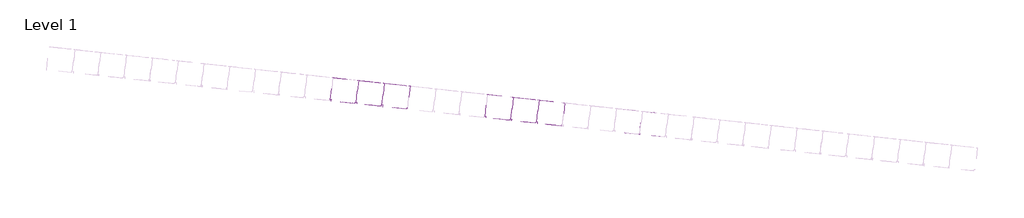
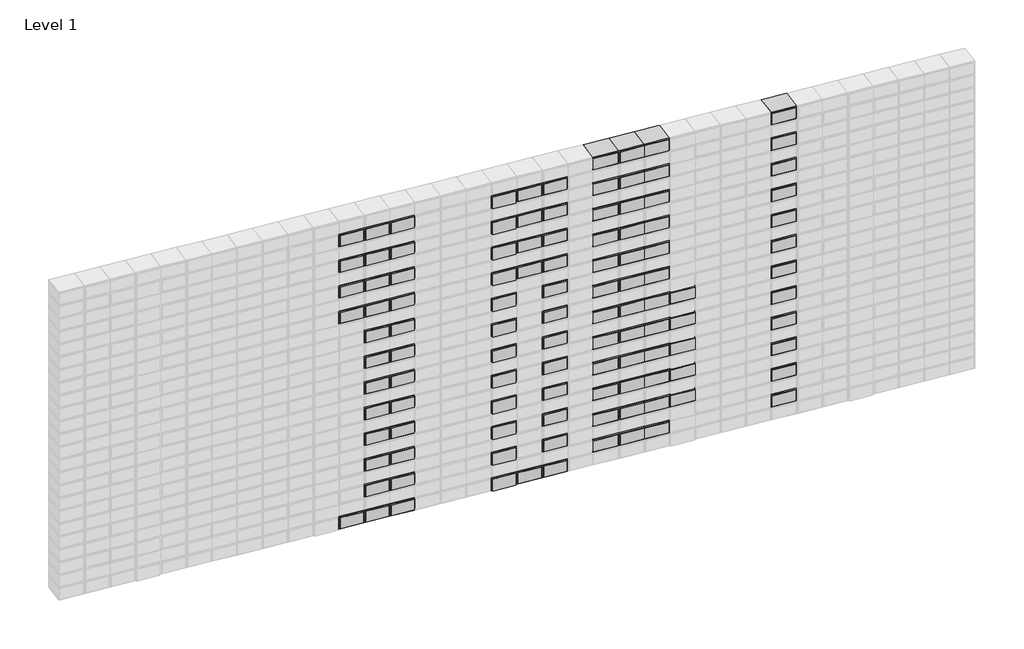
# One storey, part 15 of 18: 111 proxies.
"""IFC4 building model written with IfcOpenShell, lengths in millimetres."""

import ifcopenshell
import ifcopenshell.guid

model = None  # the IFC model being written
_history = None  # IfcOwnerHistory: only IFC2X3 demands one
_inside = {}  # id of a spatial element -> (the spatial element, [elements in it])
_under = {}  # id of a project, library or spatial element -> (it, [spatial elements below it])
_declared = {}  # id of a project -> (the project, [libraries it declares])
_typed = {}  # id of a type object -> (the type object, [elements of that type])
_made_of = {}  # id of a material, layer set ... -> (it, [elements and type objects made of it])


def new_model(schema):
    """Start an empty IFC model of exactly this schema.

    Asked for "IFC4X3", IfcOpenShell would pick the latest addendum, in which some entities
    have other attributes; the version numbers below select the first issue.
    IFC2X3 requires an IfcOwnerHistory on every rooted entity: one is made here for all.
    """
    global model, _history
    if schema == "IFC4X3":
        model = ifcopenshell.file(schema_version=(4, 3, 0, 0))
    else:
        model = ifcopenshell.file(schema=schema)
    _inside.clear()
    _under.clear()
    _declared.clear()
    _typed.clear()
    _made_of.clear()
    _history = None
    if model.schema == "IFC2X3":
        org = make("IfcOrganization", Name="unknown")
        user = make(
            "IfcPersonAndOrganization",
            ThePerson=make("IfcPerson", FamilyName="unknown"),
            TheOrganization=org,
        )
        app = make(
            "IfcApplication",
            ApplicationDeveloper=org,
            Version="unknown",
            ApplicationFullName="unknown",
            ApplicationIdentifier="unknown",
        )
        _history = make(
            "IfcOwnerHistory",
            OwningUser=user,
            OwningApplication=app,
            ChangeAction="ADDED",
            CreationDate=0,
        )
    return model


def make(cls, **values):
    """One entity of the class cls with the attributes given. An attribute that is None is left unset."""
    return model.create_entity(
        cls, **{name: value for name, value in values.items() if value is not None}
    )


def rooted(cls, **values):
    """An entity with a GlobalId (a new one), such as an element, a storey or a relation."""
    return make(cls, GlobalId=ifcopenshell.guid.new(), OwnerHistory=_history, **values)


def si_unit(unit_type, name, prefix=None):
    """IfcSIUnit, for example si_unit("LENGTHUNIT", "METRE", prefix="MILLI")."""
    return make("IfcSIUnit", UnitType=unit_type, Prefix=prefix, Name=name)


def assignment(units):
    """IfcUnitAssignment: the units of a project."""
    return None if units is None else make("IfcUnitAssignment", Units=units)


def point(xyz):
    """IfcCartesianPoint."""
    return None if xyz is None else make("IfcCartesianPoint", Coordinates=xyz)


def direction(xyz):
    """IfcDirection."""
    return None if xyz is None else make("IfcDirection", DirectionRatios=xyz)


def frame(location, z_axis=None, x_axis=None):
    """IfcAxis2Placement3D, a coordinate frame: its origin and axes. An axis left out is left unset."""
    return make(
        "IfcAxis2Placement3D",
        Location=point(location),
        Axis=direction(z_axis),
        RefDirection=direction(x_axis),
    )


def origin():
    """The frame at (0, 0, 0) with its axes left unset."""
    return frame((0.0, 0.0, 0.0))


def origin_with_axes():
    """The frame at (0, 0, 0) with the z axis (0, 0, 1) and the x axis (1, 0, 0) written out."""
    return frame((0.0, 0.0, 0.0), z_axis=(0.0, 0.0, 1.0), x_axis=(1.0, 0.0, 0.0))


def place(relative_to, where):
    """IfcLocalPlacement: puts the frame where relative to a parent placement (None: the world)."""
    return make(
        "IfcLocalPlacement", PlacementRelTo=relative_to, RelativePlacement=where
    )


def context(
    kind, dimensions, precision=None, world=None, true_north=None, identifier=None
):
    """IfcGeometricRepresentationContext, for example the 3D "Model" context."""
    return make(
        "IfcGeometricRepresentationContext",
        ContextIdentifier=identifier,
        ContextType=kind,
        CoordinateSpaceDimension=dimensions,
        Precision=precision,
        WorldCoordinateSystem=world,
        TrueNorth=true_north,
    )


def project(units=None, contexts=None):
    """IfcProject with its units and contexts."""
    return rooted(
        "IfcProject",
        Name="project",
        RepresentationContexts=contexts,
        UnitsInContext=assignment(units),
    )


def spatial(cls, under=None, at=None, **own):
    """A site, building, storey or space (cls), placed at a placement, below another one or the project."""
    s = rooted(cls, ObjectPlacement=at, **own)
    if under is not None:
        _under.setdefault(under.id(), (under, []))[1].append(s)
    return s


def polyline(points):
    """IfcPolyline through the points."""
    return make("IfcPolyline", Points=[point(p) for p in points])


def outline(outer, holes=None, kind="AREA"):
    """IfcArbitraryClosedProfileDef: a profile drawn as a closed curve; with holes, ...WithVoids."""
    if holes is None:
        return make("IfcArbitraryClosedProfileDef", ProfileType=kind, OuterCurve=outer)
    return make(
        "IfcArbitraryProfileDefWithVoids",
        ProfileType=kind,
        OuterCurve=outer,
        InnerCurves=holes,
    )


def extrude(swept, where, along, depth):
    """IfcExtrudedAreaSolid: the profile swept, set in the frame where, extruded along a direction by depth."""
    return make(
        "IfcExtrudedAreaSolid",
        SweptArea=swept,
        Position=where,
        ExtrudedDirection=direction(along),
        Depth=depth,
    )


def shape(context_of_items, identifier, shape_type, items):
    """IfcShapeRepresentation: the items that make up one representation, for example the "Body"."""
    return make(
        "IfcShapeRepresentation",
        ContextOfItems=context_of_items,
        RepresentationIdentifier=identifier,
        RepresentationType=shape_type,
        Items=items,
    )


def source(mapping_origin, context_of_items, identifier, shape_type, items):
    """IfcRepresentationMap: a shape defined once, which mapped items show again and again."""
    return make(
        "IfcRepresentationMap",
        MappingOrigin=mapping_origin,
        MappedRepresentation=shape(context_of_items, identifier, shape_type, items),
    )


def transform(
    local_origin,
    x_axis=None,
    y_axis=None,
    z_axis=None,
    scale=None,
    scale2=None,
    scale3=None,
    uniform=True,
):
    """IfcCartesianTransformationOperator3D, or its non-uniform kind. x_axis, y_axis, z_axis: its Axis1, 2, 3."""
    if uniform:
        return make(
            "IfcCartesianTransformationOperator3D",
            Axis1=direction(x_axis),
            Axis2=direction(y_axis),
            LocalOrigin=point(local_origin),
            Scale=scale,
            Axis3=direction(z_axis),
        )
    return make(
        "IfcCartesianTransformationOperator3DnonUniform",
        Axis1=direction(x_axis),
        Axis2=direction(y_axis),
        LocalOrigin=point(local_origin),
        Scale=scale,
        Axis3=direction(z_axis),
        Scale2=scale2,
        Scale3=scale3,
    )


def mapped(mapping_source, mapping_target):
    """IfcMappedItem: shows the shape of a source again, moved by a transform."""
    return make(
        "IfcMappedItem", MappingSource=mapping_source, MappingTarget=mapping_target
    )


def made_of(thing, what):
    """Note that an element or type object is made of a material, layer set ...; save() writes the relation."""
    if what is not None:
        _made_of.setdefault(what.id(), (what, []))[1].append(thing)
    return thing


def element(
    cls,
    number,
    at=None,
    inside=None,
    cuts=None,
    type_object=None,
    material=None,
    context=None,
    identifier="Body",
    shape_type=None,
    held_by="IfcProductDefinitionShape",
    body=None,
    shapes=None,
    **own,
):
    """One element of the class cls, such as IfcWall. Its Tag is "e" and its number.

    at: its placement. inside: the storey or other place that contains it. cuts: it is an
    opening in that element (IfcRelVoidsElement). A single representation is given by context,
    identifier, shape_type and body (its items); several are given by shapes. held_by: the class
    of the entity that holds the representations. save() writes the other relations.
    """
    e = rooted(cls, Tag="e%d" % number, ObjectPlacement=at, **own)
    if body is not None:
        shapes = [shape(context, identifier, shape_type, body)]
    if shapes is not None:
        e.Representation = make(held_by, Representations=shapes)
    if inside is not None:
        _inside.setdefault(inside.id(), (inside, []))[1].append(e)
    if cuts is not None:
        rooted(
            "IfcRelVoidsElement", RelatingBuildingElement=cuts, RelatedOpeningElement=e
        )
    if type_object is not None:
        _typed.setdefault(type_object.id(), (type_object, []))[1].append(e)
    return made_of(e, material)


def aggregate(whole, parts):
    """IfcRelAggregates: a whole, such as a stair, and the parts it consists of."""
    return rooted("IfcRelAggregates", RelatingObject=whole, RelatedObjects=parts)


def save(model, path):
    """Write the relations noted so far, then the file.

    IfcRelAggregates (storeys below a building ...), IfcRelContainedInSpatialStructure (elements
    in a storey), IfcRelDefinesByType, IfcRelAssociatesMaterial and IfcRelDeclares: one each for
    every whole, place, type object, material and project.
    """
    for whole, parts in _under.values():
        aggregate(whole, parts)
    for where, things in _inside.values():
        rooted(
            "IfcRelContainedInSpatialStructure",
            RelatedElements=things,
            RelatingStructure=where,
        )
    for kind, things in _typed.values():
        rooted("IfcRelDefinesByType", RelatedObjects=things, RelatingType=kind)
    for what, things in _made_of.values():
        rooted("IfcRelAssociatesMaterial", RelatedObjects=things, RelatingMaterial=what)
    for by, libraries in _declared.values():
        rooted("IfcRelDeclares", RelatingContext=by, RelatedDefinitions=libraries)
    model.write(path)


def geel_a5fc7152(model_context):
    return source(origin(), model_context, "Body", "SweptSolid", [
        extrude(outline(polyline([(131.1871262, 51.8695461), (24.8461542, 24.0369432), (23.5801491, 28.8740117), (125.0840527, 55.4406095), (111.9430518, 105.6488784), (10.4391482, 79.0822806), (9.1731432, 83.919349), (115.5141152, 111.7519519), (131.1871262, 51.8695461)])), origin_with_axes(), (0.0, 0.0, 1.0), 95.0),
        extrude(outline(polyline([(111.9430518, 105.6488784), (125.0840527, 55.4406095), (23.5801491, 28.8740117), (10.4391482, 79.0822806), (111.9430518, 105.6488784)])), origin_with_axes(), (0.0, 0.0, 1.0), 100.0),
    ])


def geel_ff5a4212(model_context):
    return source(origin(), model_context, "Body", "SweptSolid", [
        extrude(outline(polyline([(24.8461542, 24.0369432), (9.1731432, 83.919349), (115.5141152, 111.7519519), (116.7801202, 106.9148835), (15.2762167, 80.3482856), (28.4172176, 30.1400167), (129.9211211, 56.7066146), (131.1871262, 51.8695461), (24.8461542, 24.0369432)])), origin_with_axes(), (0.0, 0.0, 1.0), 95.0),
        extrude(outline(polyline([(116.7801202, 106.9148835), (129.9211211, 56.7066146), (28.4172176, 30.1400167), (15.2762167, 80.3482856), (116.7801202, 106.9148835)])), origin_with_axes(), (0.0, 0.0, 1.0), 100.0),
    ])


def rood_14a66368(model_context):
    return source(origin(), model_context, "Body", "SweptSolid", [
        extrude(outline(polyline([(24.8461542, 24.0369432), (9.1731432, 83.919349), (115.5141152, 111.7519519), (131.1871262, 51.8695461), (24.8461542, 24.0369432)]), holes=[polyline([(125.0840527, 55.4406095), (111.9430518, 105.6488784), (15.2762167, 80.3482856), (28.4172176, 30.1400167), (125.0840527, 55.4406095)])]), origin_with_axes(), (0.0, 0.0, 1.0), 95.0),
        extrude(outline(polyline([(111.9430518, 105.6488784), (125.0840527, 55.4406095), (28.4172176, 30.1400167), (15.2762167, 80.3482856), (111.9430518, 105.6488784)])), origin_with_axes(), (0.0, 0.0, 1.0), 100.0),
    ])


def rood_2ddd8018(model_context):
    return source(origin(), model_context, "Body", "SweptSolid", [
        extrude(outline(polyline([(24.8461542, 24.0369432), (9.1731432, 83.919349), (115.5141152, 111.7519519), (131.1871262, 51.8695461), (126.3500577, 50.6035411), (111.9430518, 105.6488784), (15.2762167, 80.3482856), (29.6832226, 25.3029482), (24.8461542, 24.0369432)])), origin_with_axes(), (0.0, 0.0, 1.0), 95.0),
        extrude(outline(polyline([(111.9430518, 105.6488784), (126.3500577, 50.6035411), (29.6832226, 25.3029482), (15.2762167, 80.3482856), (111.9430518, 105.6488784)])), origin_with_axes(), (0.0, 0.0, 1.0), 100.0),
    ])


model = new_model("IFC4")

# Units and contexts
model_context = context("Model", 3, world=origin())
ifc_project = project(units=[si_unit("LENGTHUNIT", "METRE", prefix="MILLI")], contexts=[model_context])

# Site, building, storey
site = spatial("IfcSite", under=ifc_project)
building = spatial("IfcBuilding", under=site)
storey = spatial("IfcBuildingStorey", under=building, Name="Level 1", Elevation=0.0)

# Proxies
placement = place(None, origin())
geel_shape = geel_a5fc7152(model_context)
element("IfcBuildingElementProxy", 1, Name="Geel", ObjectType="Geel", at=placement, inside=storey, context=model_context, shape_type="MappedRepresentation", body=[
    mapped(geel_shape, transform((11171.9037428, -4526.1762984, 2168.7358475), x_axis=(0.9617275503729374, -0.1047347566147725, -0.25320100633787673), y_axis=(0.25171277368869216, -0.02741220845642974, 0.9674136914420255), z_axis=(-0.10826263628609081, -0.9941223272738551, 0.0))),
])
element("IfcBuildingElementProxy", 2, Name="Geel", ObjectType="Geel", at=placement, inside=storey, context=model_context, shape_type="MappedRepresentation", body=[
    mapped(geel_shape, transform((11936.8417921, -4609.4801409, 2168.7358475), x_axis=(0.9617275503729374, -0.10473475661477244, -0.25320100633787673), y_axis=(0.25171277368869216, -0.027412208456429728, 0.9674136914420255), z_axis=(-0.10826263628609079, -0.9941223272738551, 0.0))),
])
element("IfcBuildingElementProxy", 3, Name="Geel", ObjectType="Geel", at=placement, inside=storey, context=model_context, shape_type="MappedRepresentation", body=[
    mapped(geel_shape, transform((11171.9037428, -4526.1762984, 2292.5348104), x_axis=(0.9617275503729374, -0.1047347566147725, -0.25320100633787673), y_axis=(0.25171277368869216, -0.02741220845642974, 0.9674136914420255), z_axis=(-0.10826263628609081, -0.9941223272738551, 0.0))),
])
element("IfcBuildingElementProxy", 4, Name="Geel", ObjectType="Geel", at=placement, inside=storey, context=model_context, shape_type="MappedRepresentation", body=[
    mapped(geel_shape, transform((11936.8417921, -4609.4801409, 2292.5348104), x_axis=(0.9617275503729374, -0.10473475661477244, -0.25320100633787673), y_axis=(0.25171277368869216, -0.027412208456429728, 0.9674136914420255), z_axis=(-0.10826263628609079, -0.9941223272738551, 0.0))),
])
element("IfcBuildingElementProxy", 5, Name="Geel", ObjectType="Geel", at=placement, inside=storey, context=model_context, shape_type="MappedRepresentation", body=[
    mapped(geel_shape, transform((11171.9037428, -4526.1762984, 2416.3337732), x_axis=(0.9617275503729384, -0.1047347566147726, -0.25320100633787307), y_axis=(0.25171277368868855, -0.02741220845642934, 0.9674136914420265), z_axis=(-0.10826263628609081, -0.994122327273855, 0.0))),
])
element("IfcBuildingElementProxy", 6, Name="Geel", ObjectType="Geel", at=placement, inside=storey, context=model_context, shape_type="MappedRepresentation", body=[
    mapped(geel_shape, transform((11936.8417921, -4609.4801409, 2416.3337732), x_axis=(0.9617275503729384, -0.10473475661477255, -0.25320100633787307), y_axis=(0.25171277368868855, -0.027412208456429325, 0.9674136914420265), z_axis=(-0.10826263628609077, -0.994122327273855, 0.0))),
])
element("IfcBuildingElementProxy", 7, Name="Geel", ObjectType="Geel", at=placement, inside=storey, context=model_context, shape_type="MappedRepresentation", body=[
    mapped(geel_shape, transform((11171.9037428, -4526.1762984, 2540.132736), x_axis=(0.9617275503729374, -0.1047347566147725, -0.25320100633787673), y_axis=(0.25171277368869216, -0.02741220845642974, 0.9674136914420255), z_axis=(-0.10826263628609081, -0.9941223272738551, 0.0))),
])
element("IfcBuildingElementProxy", 8, Name="Geel", ObjectType="Geel", at=placement, inside=storey, context=model_context, shape_type="MappedRepresentation", body=[
    mapped(geel_shape, transform((11936.8417921, -4609.4801409, 2540.132736), x_axis=(0.9617275503729374, -0.10473475661477244, -0.25320100633787673), y_axis=(0.25171277368869216, -0.027412208456429728, 0.9674136914420255), z_axis=(-0.10826263628609079, -0.9941223272738551, 0.0))),
])
element("IfcBuildingElementProxy", 9, Name="Geel", ObjectType="Geel", at=placement, inside=storey, context=model_context, shape_type="MappedRepresentation", body=[
    mapped(geel_shape, transform((11171.9037428, -4526.1762984, 2663.9316989), x_axis=(0.9617275503729374, -0.1047347566147725, -0.25320100633787673), y_axis=(0.25171277368869216, -0.02741220845642974, 0.9674136914420255), z_axis=(-0.10826263628609081, -0.9941223272738551, 0.0))),
])
element("IfcBuildingElementProxy", 10, Name="Geel", ObjectType="Geel", at=placement, inside=storey, context=model_context, shape_type="MappedRepresentation", body=[
    mapped(geel_shape, transform((11936.8417921, -4609.4801409, 2663.9316989), x_axis=(0.9617275503729374, -0.10473475661477244, -0.25320100633787673), y_axis=(0.25171277368869216, -0.027412208456429728, 0.9674136914420255), z_axis=(-0.10826263628609079, -0.9941223272738551, 0.0))),
])
element("IfcBuildingElementProxy", 11, Name="Geel", ObjectType="Geel", at=placement, inside=storey, context=model_context, shape_type="MappedRepresentation", body=[
    mapped(geel_shape, transform((11171.9037428, -4526.1762984, 2787.7306617), x_axis=(0.9617275503729374, -0.1047347566147725, -0.25320100633787673), y_axis=(0.25171277368869216, -0.02741220845642974, 0.9674136914420255), z_axis=(-0.10826263628609081, -0.9941223272738551, 0.0))),
])
element("IfcBuildingElementProxy", 12, Name="Geel", ObjectType="Geel", at=placement, inside=storey, context=model_context, shape_type="MappedRepresentation", body=[
    mapped(geel_shape, transform((11936.8417921, -4609.4801409, 2787.7306617), x_axis=(0.9617275503729374, -0.10473475661477244, -0.25320100633787673), y_axis=(0.25171277368869216, -0.027412208456429728, 0.9674136914420255), z_axis=(-0.10826263628609079, -0.9941223272738551, 0.0))),
])
element("IfcBuildingElementProxy", 13, Name="Geel", ObjectType="Geel", at=placement, inside=storey, context=model_context, shape_type="MappedRepresentation", body=[
    mapped(geel_shape, transform((11171.9037428, -4526.1762984, 2911.5296245), x_axis=(0.9617275503729374, -0.1047347566147725, -0.25320100633787673), y_axis=(0.25171277368869216, -0.02741220845642974, 0.9674136914420255), z_axis=(-0.10826263628609081, -0.9941223272738551, 0.0))),
])
element("IfcBuildingElementProxy", 14, Name="Geel", ObjectType="Geel", at=placement, inside=storey, context=model_context, shape_type="MappedRepresentation", body=[
    mapped(geel_shape, transform((11936.8417921, -4609.4801409, 2911.5296245), x_axis=(0.9617275503729374, -0.10473475661477244, -0.25320100633787673), y_axis=(0.25171277368869216, -0.027412208456429728, 0.9674136914420255), z_axis=(-0.10826263628609079, -0.9941223272738551, 0.0))),
])
element("IfcBuildingElementProxy", 15, Name="Geel", ObjectType="Geel", at=placement, inside=storey, context=model_context, shape_type="MappedRepresentation", body=[
    mapped(geel_shape, transform((11171.9037428, -4526.1762984, 3035.3285874), x_axis=(0.9617275503729374, -0.1047347566147725, -0.25320100633787673), y_axis=(0.25171277368869216, -0.02741220845642974, 0.9674136914420255), z_axis=(-0.10826263628609081, -0.9941223272738551, 0.0))),
])
element("IfcBuildingElementProxy", 16, Name="Geel", ObjectType="Geel", at=placement, inside=storey, context=model_context, shape_type="MappedRepresentation", body=[
    mapped(geel_shape, transform((11936.8417921, -4609.4801409, 3035.3285874), x_axis=(0.9617275503729374, -0.10473475661477244, -0.25320100633787673), y_axis=(0.25171277368869216, -0.027412208456429728, 0.9674136914420255), z_axis=(-0.10826263628609079, -0.9941223272738551, 0.0))),
])
element("IfcBuildingElementProxy", 17, Name="Geel", ObjectType="Geel", at=placement, inside=storey, context=model_context, shape_type="MappedRepresentation", body=[
    mapped(geel_shape, transform((11171.9037428, -4526.1762984, 3159.1275502), x_axis=(0.9617275503729374, -0.1047347566147725, -0.25320100633787673), y_axis=(0.25171277368869216, -0.02741220845642974, 0.9674136914420255), z_axis=(-0.10826263628609081, -0.9941223272738551, 0.0))),
])
element("IfcBuildingElementProxy", 18, Name="Geel", ObjectType="Geel", at=placement, inside=storey, context=model_context, shape_type="MappedRepresentation", body=[
    mapped(geel_shape, transform((11936.8417921, -4609.4801409, 3159.1275502), x_axis=(0.9617275503729374, -0.10473475661477244, -0.25320100633787673), y_axis=(0.25171277368869216, -0.027412208456429728, 0.9674136914420255), z_axis=(-0.10826263628609079, -0.9941223272738551, 0.0))),
])
element("IfcBuildingElementProxy", 19, Name="Geel", ObjectType="Geel", at=placement, inside=storey, context=model_context, shape_type="MappedRepresentation", body=[
    mapped(geel_shape, transform((11171.9037428, -4526.1762984, 3282.926513), x_axis=(0.9617275503729374, -0.1047347566147725, -0.25320100633787673), y_axis=(0.25171277368869216, -0.02741220845642974, 0.9674136914420255), z_axis=(-0.10826263628609081, -0.9941223272738551, 0.0))),
])
element("IfcBuildingElementProxy", 20, Name="Geel", ObjectType="Geel", at=placement, inside=storey, context=model_context, shape_type="MappedRepresentation", body=[
    mapped(geel_shape, transform((11936.8417921, -4609.4801409, 3282.926513), x_axis=(0.9617275503729374, -0.10473475661477244, -0.25320100633787673), y_axis=(0.25171277368869216, -0.027412208456429728, 0.9674136914420255), z_axis=(-0.10826263628609079, -0.9941223272738551, 0.0))),
])
element("IfcBuildingElementProxy", 21, Name="Geel", ObjectType="Geel", at=placement, inside=storey, context=model_context, shape_type="MappedRepresentation", body=[
    mapped(geel_shape, transform((11171.9037428, -4526.1762984, 3406.7254759), x_axis=(0.9617275503729374, -0.1047347566147725, -0.25320100633787673), y_axis=(0.25171277368869216, -0.02741220845642974, 0.9674136914420255), z_axis=(-0.10826263628609081, -0.9941223272738551, 0.0))),
])
element("IfcBuildingElementProxy", 22, Name="Geel", ObjectType="Geel", at=placement, inside=storey, context=model_context, shape_type="MappedRepresentation", body=[
    mapped(geel_shape, transform((11936.8417921, -4609.4801409, 3406.7254759), x_axis=(0.9617275503729374, -0.10473475661477244, -0.25320100633787673), y_axis=(0.25171277368869216, -0.027412208456429728, 0.9674136914420255), z_axis=(-0.10826263628609079, -0.9941223272738551, 0.0))),
])
element("IfcBuildingElementProxy", 23, Name="Geel", ObjectType="Geel", at=placement, inside=storey, context=model_context, shape_type="MappedRepresentation", body=[
    mapped(geel_shape, transform((11171.9037428, -4526.1762984, 2044.9368847), x_axis=(0.9617275503729384, -0.1047347566147726, -0.25320100633787307), y_axis=(0.25171277368868855, -0.02741220845642934, 0.9674136914420265), z_axis=(-0.10826263628609081, -0.994122327273855, 0.0))),
])
element("IfcBuildingElementProxy", 24, Name="Geel", ObjectType="Geel", at=placement, inside=storey, context=model_context, shape_type="MappedRepresentation", body=[
    mapped(geel_shape, transform((11936.8417921, -4609.4801409, 2044.9368847), x_axis=(0.9617275503729384, -0.10473475661477255, -0.25320100633787307), y_axis=(0.25171277368868855, -0.027412208456429325, 0.9674136914420265), z_axis=(-0.10826263628609077, -0.994122327273855, 0.0))),
])
element("IfcBuildingElementProxy", 25, Name="Geel", ObjectType="Geel", at=placement, inside=storey, context=model_context, shape_type="MappedRepresentation", body=[
    mapped(geel_shape, transform((11390.4574712, -4549.9773962, 2168.7358475), x_axis=(0.9617275503729372, -0.1047347566147745, -0.2532010063378768), y_axis=(0.2517127736886921, -0.02741220845643024, 0.9674136914420256), z_axis=(-0.10826263628609285, -0.9941223272738547, 0.0))),
])
element("IfcBuildingElementProxy", 26, Name="Geel", ObjectType="Geel", at=placement, inside=storey, context=model_context, shape_type="MappedRepresentation", body=[
    mapped(geel_shape, transform((11390.4574712, -4549.9773962, 2292.5348104), x_axis=(0.9617275503729372, -0.1047347566147745, -0.2532010063378768), y_axis=(0.2517127736886921, -0.02741220845643024, 0.9674136914420256), z_axis=(-0.10826263628609285, -0.9941223272738547, 0.0))),
])
element("IfcBuildingElementProxy", 27, Name="Geel", ObjectType="Geel", at=placement, inside=storey, context=model_context, shape_type="MappedRepresentation", body=[
    mapped(geel_shape, transform((11390.4574712, -4549.9773962, 2416.3337732), x_axis=(0.9617275503729381, -0.10473475661477456, -0.2532010063378731), y_axis=(0.2517127736886886, -0.02741220845642988, 0.9674136914420264), z_axis=(-0.10826263628609287, -0.9941223272738549, 0.0))),
])
element("IfcBuildingElementProxy", 28, Name="Geel", ObjectType="Geel", at=placement, inside=storey, context=model_context, shape_type="MappedRepresentation", body=[
    mapped(geel_shape, transform((11390.4574712, -4549.9773962, 2540.132736), x_axis=(0.9617275503729372, -0.1047347566147745, -0.2532010063378768), y_axis=(0.2517127736886921, -0.02741220845643024, 0.9674136914420256), z_axis=(-0.10826263628609285, -0.9941223272738547, 0.0))),
])
element("IfcBuildingElementProxy", 29, Name="Geel", ObjectType="Geel", at=placement, inside=storey, context=model_context, shape_type="MappedRepresentation", body=[
    mapped(geel_shape, transform((11390.4574712, -4549.9773962, 2663.9316989), x_axis=(0.9617275503729372, -0.1047347566147745, -0.2532010063378768), y_axis=(0.2517127736886921, -0.02741220845643024, 0.9674136914420256), z_axis=(-0.10826263628609285, -0.9941223272738547, 0.0))),
])
element("IfcBuildingElementProxy", 30, Name="Geel", ObjectType="Geel", at=placement, inside=storey, context=model_context, shape_type="MappedRepresentation", body=[
    mapped(geel_shape, transform((11390.4574712, -4549.9773962, 2787.7306617), x_axis=(0.9617275503729372, -0.1047347566147745, -0.2532010063378768), y_axis=(0.2517127736886921, -0.02741220845643024, 0.9674136914420256), z_axis=(-0.10826263628609285, -0.9941223272738547, 0.0))),
])
element("IfcBuildingElementProxy", 31, Name="Geel", ObjectType="Geel", at=placement, inside=storey, context=model_context, shape_type="MappedRepresentation", body=[
    mapped(geel_shape, transform((11390.4574712, -4549.9773962, 2911.5296245), x_axis=(0.9617275503729372, -0.1047347566147745, -0.2532010063378768), y_axis=(0.2517127736886921, -0.02741220845643024, 0.9674136914420256), z_axis=(-0.10826263628609285, -0.9941223272738547, 0.0))),
])
element("IfcBuildingElementProxy", 32, Name="Geel", ObjectType="Geel", at=placement, inside=storey, context=model_context, shape_type="MappedRepresentation", body=[
    mapped(geel_shape, transform((11390.4574712, -4549.9773962, 3035.3285874), x_axis=(0.9617275503729372, -0.1047347566147745, -0.2532010063378768), y_axis=(0.2517127736886921, -0.02741220845643024, 0.9674136914420256), z_axis=(-0.10826263628609285, -0.9941223272738547, 0.0))),
])
element("IfcBuildingElementProxy", 33, Name="Geel", ObjectType="Geel", at=placement, inside=storey, context=model_context, shape_type="MappedRepresentation", body=[
    mapped(geel_shape, transform((11390.4574712, -4549.9773962, 3159.1275502), x_axis=(0.9617275503729372, -0.1047347566147745, -0.2532010063378768), y_axis=(0.2517127736886921, -0.02741220845643024, 0.9674136914420256), z_axis=(-0.10826263628609285, -0.9941223272738547, 0.0))),
])
element("IfcBuildingElementProxy", 34, Name="Geel", ObjectType="Geel", at=placement, inside=storey, context=model_context, shape_type="MappedRepresentation", body=[
    mapped(geel_shape, transform((11390.4574712, -4549.9773962, 3282.926513), x_axis=(0.9617275503729372, -0.1047347566147745, -0.2532010063378768), y_axis=(0.2517127736886921, -0.02741220845643024, 0.9674136914420256), z_axis=(-0.10826263628609285, -0.9941223272738547, 0.0))),
])
element("IfcBuildingElementProxy", 35, Name="Geel", ObjectType="Geel", at=placement, inside=storey, context=model_context, shape_type="MappedRepresentation", body=[
    mapped(geel_shape, transform((11390.4574712, -4549.9773962, 3406.7254759), x_axis=(0.9617275503729372, -0.1047347566147745, -0.2532010063378768), y_axis=(0.2517127736886921, -0.02741220845643024, 0.9674136914420256), z_axis=(-0.10826263628609285, -0.9941223272738547, 0.0))),
])
element("IfcBuildingElementProxy", 36, Name="Geel", ObjectType="Geel", at=placement, inside=storey, context=model_context, shape_type="MappedRepresentation", body=[
    mapped(geel_shape, transform((11390.4574712, -4549.9773962, 2044.9368847), x_axis=(0.9617275503729381, -0.10473475661477456, -0.2532010063378731), y_axis=(0.2517127736886886, -0.02741220845642988, 0.9674136914420264), z_axis=(-0.10826263628609287, -0.9941223272738549, 0.0))),
])
geel_2_shape = geel_ff5a4212(model_context)
element("IfcBuildingElementProxy", 37, Name="Geel", ObjectType="Geel", at=placement, inside=storey, context=model_context, shape_type="MappedRepresentation", body=[
    mapped(geel_2_shape, transform((11281.180607, -4538.0768473, 2168.7358475), x_axis=(0.9617275503729374, -0.1047347566147725, -0.25320100633787673), y_axis=(0.25171277368869216, -0.02741220845642974, 0.9674136914420255), z_axis=(-0.10826263628609081, -0.9941223272738551, 0.0))),
])
element("IfcBuildingElementProxy", 38, Name="Geel", ObjectType="Geel", at=placement, inside=storey, context=model_context, shape_type="MappedRepresentation", body=[
    mapped(geel_2_shape, transform((11281.180607, -4538.0768473, 2292.5348104), x_axis=(0.9617275503729374, -0.1047347566147725, -0.25320100633787673), y_axis=(0.25171277368869216, -0.02741220845642974, 0.9674136914420255), z_axis=(-0.10826263628609081, -0.9941223272738551, 0.0))),
])
element("IfcBuildingElementProxy", 39, Name="Geel", ObjectType="Geel", at=placement, inside=storey, context=model_context, shape_type="MappedRepresentation", body=[
    mapped(geel_2_shape, transform((11281.180607, -4538.0768473, 2416.3337732), x_axis=(0.9617275503729384, -0.1047347566147726, -0.25320100633787307), y_axis=(0.25171277368868855, -0.02741220845642934, 0.9674136914420265), z_axis=(-0.10826263628609081, -0.994122327273855, 0.0))),
])
element("IfcBuildingElementProxy", 40, Name="Geel", ObjectType="Geel", at=placement, inside=storey, context=model_context, shape_type="MappedRepresentation", body=[
    mapped(geel_2_shape, transform((11281.180607, -4538.0768473, 2540.132736), x_axis=(0.9617275503729374, -0.1047347566147725, -0.25320100633787673), y_axis=(0.25171277368869216, -0.02741220845642974, 0.9674136914420255), z_axis=(-0.10826263628609081, -0.9941223272738551, 0.0))),
])
element("IfcBuildingElementProxy", 41, Name="Geel", ObjectType="Geel", at=placement, inside=storey, context=model_context, shape_type="MappedRepresentation", body=[
    mapped(geel_2_shape, transform((11281.180607, -4538.0768473, 2663.9316989), x_axis=(0.9617275503729374, -0.1047347566147725, -0.25320100633787673), y_axis=(0.25171277368869216, -0.02741220845642974, 0.9674136914420255), z_axis=(-0.10826263628609081, -0.9941223272738551, 0.0))),
])
element("IfcBuildingElementProxy", 42, Name="Geel", ObjectType="Geel", at=placement, inside=storey, context=model_context, shape_type="MappedRepresentation", body=[
    mapped(geel_2_shape, transform((11281.180607, -4538.0768473, 2787.7306617), x_axis=(0.9617275503729374, -0.1047347566147725, -0.25320100633787673), y_axis=(0.25171277368869216, -0.02741220845642974, 0.9674136914420255), z_axis=(-0.10826263628609081, -0.9941223272738551, 0.0))),
])
element("IfcBuildingElementProxy", 43, Name="Geel", ObjectType="Geel", at=placement, inside=storey, context=model_context, shape_type="MappedRepresentation", body=[
    mapped(geel_2_shape, transform((11281.180607, -4538.0768473, 2911.5296245), x_axis=(0.9617275503729374, -0.1047347566147725, -0.25320100633787673), y_axis=(0.25171277368869216, -0.02741220845642974, 0.9674136914420255), z_axis=(-0.10826263628609081, -0.9941223272738551, 0.0))),
])
element("IfcBuildingElementProxy", 44, Name="Geel", ObjectType="Geel", at=placement, inside=storey, context=model_context, shape_type="MappedRepresentation", body=[
    mapped(geel_2_shape, transform((11281.180607, -4538.0768473, 3035.3285874), x_axis=(0.9617275503729374, -0.1047347566147725, -0.25320100633787673), y_axis=(0.25171277368869216, -0.02741220845642974, 0.9674136914420255), z_axis=(-0.10826263628609081, -0.9941223272738551, 0.0))),
])
element("IfcBuildingElementProxy", 45, Name="Geel", ObjectType="Geel", at=placement, inside=storey, context=model_context, shape_type="MappedRepresentation", body=[
    mapped(geel_2_shape, transform((11281.180607, -4538.0768473, 3159.1275502), x_axis=(0.9617275503729374, -0.1047347566147725, -0.25320100633787673), y_axis=(0.25171277368869216, -0.02741220845642974, 0.9674136914420255), z_axis=(-0.10826263628609081, -0.9941223272738551, 0.0))),
])
element("IfcBuildingElementProxy", 46, Name="Geel", ObjectType="Geel", at=placement, inside=storey, context=model_context, shape_type="MappedRepresentation", body=[
    mapped(geel_2_shape, transform((11281.180607, -4538.0768473, 3282.926513), x_axis=(0.9617275503729374, -0.1047347566147725, -0.25320100633787673), y_axis=(0.25171277368869216, -0.02741220845642974, 0.9674136914420255), z_axis=(-0.10826263628609081, -0.9941223272738551, 0.0))),
])
element("IfcBuildingElementProxy", 47, Name="Geel", ObjectType="Geel", at=placement, inside=storey, context=model_context, shape_type="MappedRepresentation", body=[
    mapped(geel_2_shape, transform((11281.180607, -4538.0768473, 3406.7254759), x_axis=(0.9617275503729374, -0.1047347566147725, -0.25320100633787673), y_axis=(0.25171277368869216, -0.02741220845642974, 0.9674136914420255), z_axis=(-0.10826263628609081, -0.9941223272738551, 0.0))),
])
element("IfcBuildingElementProxy", 48, Name="Geel", ObjectType="Geel", at=placement, inside=storey, context=model_context, shape_type="MappedRepresentation", body=[
    mapped(geel_2_shape, transform((11281.180607, -4538.0768473, 2044.9368847), x_axis=(0.9617275503729384, -0.1047347566147726, -0.25320100633787307), y_axis=(0.25171277368868855, -0.02741220845642934, 0.9674136914420265), z_axis=(-0.10826263628609081, -0.994122327273855, 0.0))),
])
element("IfcBuildingElementProxy", 49, Name="Geel", ObjectType="Geel", at=placement, inside=storey, context=model_context, shape_type="MappedRepresentation", body=[
    mapped(geel_2_shape, transform((11499.7343354, -4561.8779452, 2168.7358475), x_axis=(0.9617275503729381, -0.10473475661476775, -0.25320100633787634), y_axis=(0.2517127736886919, -0.02741220845642843, 0.9674136914420257), z_axis=(-0.1082626362860859, -0.9941223272738555, 0.0))),
])
element("IfcBuildingElementProxy", 50, Name="Geel", ObjectType="Geel", at=placement, inside=storey, context=model_context, shape_type="MappedRepresentation", body=[
    mapped(geel_2_shape, transform((11499.7343354, -4561.8779452, 2292.5348104), x_axis=(0.9617275503729381, -0.10473475661476775, -0.25320100633787634), y_axis=(0.2517127736886919, -0.02741220845642843, 0.9674136914420257), z_axis=(-0.1082626362860859, -0.9941223272738555, 0.0))),
])
element("IfcBuildingElementProxy", 51, Name="Geel", ObjectType="Geel", at=placement, inside=storey, context=model_context, shape_type="MappedRepresentation", body=[
    mapped(geel_2_shape, transform((11499.7343354, -4561.8779452, 2416.3337732), x_axis=(0.961727550372939, -0.10473475661476785, -0.2532010063378727), y_axis=(0.2517127736886882, -0.02741220845642804, 0.9674136914420266), z_axis=(-0.1082626362860859, -0.9941223272738555, 0.0))),
])
element("IfcBuildingElementProxy", 52, Name="Geel", ObjectType="Geel", at=placement, inside=storey, context=model_context, shape_type="MappedRepresentation", body=[
    mapped(geel_2_shape, transform((11499.7343354, -4561.8779452, 2540.132736), x_axis=(0.9617275503729381, -0.10473475661476775, -0.25320100633787634), y_axis=(0.2517127736886919, -0.02741220845642843, 0.9674136914420257), z_axis=(-0.1082626362860859, -0.9941223272738555, 0.0))),
])
element("IfcBuildingElementProxy", 53, Name="Geel", ObjectType="Geel", at=placement, inside=storey, context=model_context, shape_type="MappedRepresentation", body=[
    mapped(geel_2_shape, transform((11499.7343354, -4561.8779452, 2663.9316989), x_axis=(0.9617275503729381, -0.10473475661476775, -0.25320100633787634), y_axis=(0.2517127736886919, -0.02741220845642843, 0.9674136914420257), z_axis=(-0.1082626362860859, -0.9941223272738555, 0.0))),
])
rood_shape = rood_14a66368(model_context)
element("IfcBuildingElementProxy", 54, Name="Rood", ObjectType="Rood", at=placement, inside=storey, context=model_context, shape_type="MappedRepresentation", body=[
    mapped(rood_shape, transform((10079.135101, -4407.170809, 2973.4291059), x_axis=(0.9617275503729381, -0.10473475661476775, -0.25320100633787634), y_axis=(0.2517127736886919, -0.02741220845642843, 0.9674136914420257), z_axis=(-0.1082626362860859, -0.9941223272738555, 0.0))),
])
element("IfcBuildingElementProxy", 55, Name="Rood", ObjectType="Rood", at=placement, inside=storey, context=model_context, shape_type="MappedRepresentation", body=[
    mapped(rood_shape, transform((10844.0731503, -4490.4746516, 2973.4291059), x_axis=(0.9617275503729374, -0.1047347566147725, -0.25320100633787673), y_axis=(0.25171277368869216, -0.02741220845642974, 0.9674136914420255), z_axis=(-0.10826263628609081, -0.9941223272738551, 0.0))),
])
element("IfcBuildingElementProxy", 56, Name="Rood", ObjectType="Rood", at=placement, inside=storey, context=model_context, shape_type="MappedRepresentation", body=[
    mapped(rood_shape, transform((10079.135101, -4407.170809, 3097.2280688), x_axis=(0.96172755037294, -0.10473475661476794, -0.253201006337869), y_axis=(0.2517127736886847, -0.02741220845642766, 0.9674136914420275), z_axis=(-0.1082626362860859, -0.9941223272738556, 0.0))),
])
element("IfcBuildingElementProxy", 57, Name="Rood", ObjectType="Rood", at=placement, inside=storey, context=model_context, shape_type="MappedRepresentation", body=[
    mapped(rood_shape, transform((10844.0731503, -4490.4746516, 3097.2280688), x_axis=(0.9617275503729394, -0.10473475661477268, -0.2532010063378695), y_axis=(0.2517127736886849, -0.027412208456428923, 0.9674136914420275), z_axis=(-0.1082626362860908, -0.9941223272738551, 0.0))),
])
element("IfcBuildingElementProxy", 58, Name="Rood", ObjectType="Rood", at=placement, inside=storey, context=model_context, shape_type="MappedRepresentation", body=[
    mapped(rood_shape, transform((10079.135101, -4407.170809, 3221.0270316), x_axis=(0.9617275503729381, -0.10473475661476775, -0.25320100633787634), y_axis=(0.2517127736886919, -0.02741220845642843, 0.9674136914420257), z_axis=(-0.1082626362860859, -0.9941223272738555, 0.0))),
])
element("IfcBuildingElementProxy", 59, Name="Rood", ObjectType="Rood", at=placement, inside=storey, context=model_context, shape_type="MappedRepresentation", body=[
    mapped(rood_shape, transform((10844.0731503, -4490.4746516, 3221.0270316), x_axis=(0.9617275503729374, -0.1047347566147725, -0.25320100633787673), y_axis=(0.25171277368869216, -0.02741220845642974, 0.9674136914420255), z_axis=(-0.10826263628609081, -0.9941223272738551, 0.0))),
])
element("IfcBuildingElementProxy", 60, Name="Rood", ObjectType="Rood", at=placement, inside=storey, context=model_context, shape_type="MappedRepresentation", body=[
    mapped(rood_shape, transform((10079.135101, -4407.170809, 3344.8259944), x_axis=(0.9617275503729362, -0.10473475661476758, -0.2532010063378836), y_axis=(0.2517127736886991, -0.027412208456429242, 0.9674136914420237), z_axis=(-0.10826263628608593, -0.9941223272738555, 0.0))),
])
element("IfcBuildingElementProxy", 61, Name="Rood", ObjectType="Rood", at=placement, inside=storey, context=model_context, shape_type="MappedRepresentation", body=[
    mapped(rood_shape, transform((10844.0731503, -4490.4746516, 3344.8259944), x_axis=(0.9617275503729357, -0.10473475661477229, -0.2532010063378841), y_axis=(0.2517127736886993, -0.027412208456430498, 0.9674136914420237), z_axis=(-0.10826263628609081, -0.9941223272738551, 0.0))),
])
element("IfcBuildingElementProxy", 62, Name="Rood", ObjectType="Rood", at=placement, inside=storey, context=model_context, shape_type="MappedRepresentation", body=[
    mapped(rood_shape, transform((10079.135101, -4407.170809, 1983.0374033), x_axis=(0.9617275503729381, -0.10473475661476775, -0.25320100633787634), y_axis=(0.2517127736886919, -0.02741220845642843, 0.9674136914420257), z_axis=(-0.1082626362860859, -0.9941223272738555, 0.0))),
])
element("IfcBuildingElementProxy", 63, Name="Rood", ObjectType="Rood", at=placement, inside=storey, context=model_context, shape_type="MappedRepresentation", body=[
    mapped(rood_shape, transform((10844.0731503, -4490.4746516, 1983.0374033), x_axis=(0.9617275503729374, -0.1047347566147725, -0.25320100633787673), y_axis=(0.25171277368869216, -0.02741220845642974, 0.9674136914420255), z_axis=(-0.10826263628609081, -0.9941223272738551, 0.0))),
])
element("IfcBuildingElementProxy", 64, Name="Rood", ObjectType="Rood", at=placement, inside=storey, context=model_context, shape_type="MappedRepresentation", body=[
    mapped(rood_shape, transform((10188.4119652, -4419.071358, 2106.8363661), x_axis=(0.9617275503729416, -0.10473475661477503, -0.2532010063378606), y_axis=(0.25171277368867595, -0.027412208456428513, 0.9674136914420297), z_axis=(-0.10826263628609296, -0.9941223272738547, 0.0))),
])
element("IfcBuildingElementProxy", 65, Name="Rood", ObjectType="Rood", at=placement, inside=storey, context=model_context, shape_type="MappedRepresentation", body=[
    mapped(rood_shape, transform((10953.3500145, -4502.3752005, 2106.8363661), x_axis=(0.961727550372942, -0.10473475661477023, -0.25320100633786047), y_axis=(0.2517127736886762, -0.02741220845642727, 0.9674136914420297), z_axis=(-0.10826263628608801, -0.9941223272738554, 0.0))),
])
element("IfcBuildingElementProxy", 66, Name="Rood", ObjectType="Rood", at=placement, inside=storey, context=model_context, shape_type="MappedRepresentation", body=[
    mapped(rood_shape, transform((10188.4119652, -4419.071358, 2230.6353289), x_axis=(0.9617275503729426, -0.10473475661477512, -0.253201006337857), y_axis=(0.2517127736886723, -0.027412208456428104, 0.9674136914420308), z_axis=(-0.10826263628609295, -0.9941223272738549, 0.0))),
])
element("IfcBuildingElementProxy", 67, Name="Rood", ObjectType="Rood", at=placement, inside=storey, context=model_context, shape_type="MappedRepresentation", body=[
    mapped(rood_shape, transform((10953.3500145, -4502.3752005, 2230.6353289), x_axis=(0.961727550372943, -0.10473475661477034, -0.25320100633785686), y_axis=(0.25171277368867245, -0.027412208456426876, 0.9674136914420308), z_axis=(-0.10826263628608801, -0.9941223272738553, 0.0))),
])
element("IfcBuildingElementProxy", 68, Name="Rood", ObjectType="Rood", at=placement, inside=storey, context=model_context, shape_type="MappedRepresentation", body=[
    mapped(rood_shape, transform((10188.4119652, -4419.071358, 2354.4342918), x_axis=(0.9617275503729416, -0.10473475661477503, -0.2532010063378606), y_axis=(0.25171277368867595, -0.027412208456428513, 0.9674136914420297), z_axis=(-0.10826263628609296, -0.9941223272738547, 0.0))),
])
element("IfcBuildingElementProxy", 69, Name="Rood", ObjectType="Rood", at=placement, inside=storey, context=model_context, shape_type="MappedRepresentation", body=[
    mapped(rood_shape, transform((10953.3500145, -4502.3752005, 2354.4342918), x_axis=(0.961727550372942, -0.10473475661477023, -0.25320100633786047), y_axis=(0.2517127736886762, -0.02741220845642727, 0.9674136914420297), z_axis=(-0.10826263628608801, -0.9941223272738554, 0.0))),
])
element("IfcBuildingElementProxy", 70, Name="Rood", ObjectType="Rood", at=placement, inside=storey, context=model_context, shape_type="MappedRepresentation", body=[
    mapped(rood_shape, transform((10188.4119652, -4419.071358, 2478.2332546), x_axis=(0.9617275503729416, -0.10473475661477503, -0.2532010063378606), y_axis=(0.25171277368867595, -0.027412208456428513, 0.9674136914420297), z_axis=(-0.10826263628609296, -0.9941223272738547, 0.0))),
])
element("IfcBuildingElementProxy", 71, Name="Rood", ObjectType="Rood", at=placement, inside=storey, context=model_context, shape_type="MappedRepresentation", body=[
    mapped(rood_shape, transform((10953.3500145, -4502.3752005, 2478.2332546), x_axis=(0.961727550372942, -0.10473475661477023, -0.25320100633786047), y_axis=(0.2517127736886762, -0.02741220845642727, 0.9674136914420297), z_axis=(-0.10826263628608801, -0.9941223272738554, 0.0))),
])
element("IfcBuildingElementProxy", 72, Name="Rood", ObjectType="Rood", at=placement, inside=storey, context=model_context, shape_type="MappedRepresentation", body=[
    mapped(rood_shape, transform((10188.4119652, -4419.071358, 2602.0322174), x_axis=(0.9617275503729434, -0.10473475661477524, -0.2532010063378533), y_axis=(0.25171277368866873, -0.02741220845642773, 0.9674136914420317), z_axis=(-0.10826263628609296, -0.9941223272738547, 0.0))),
])
element("IfcBuildingElementProxy", 73, Name="Rood", ObjectType="Rood", at=placement, inside=storey, context=model_context, shape_type="MappedRepresentation", body=[
    mapped(rood_shape, transform((10953.3500145, -4502.3752005, 2602.0322174), x_axis=(0.9617275503729439, -0.10473475661477047, -0.2532010063378535), y_axis=(0.2517127736886689, -0.027412208456426466, 0.9674136914420317), z_axis=(-0.10826263628608802, -0.9941223272738554, 0.0))),
])
element("IfcBuildingElementProxy", 74, Name="Rood", ObjectType="Rood", at=placement, inside=storey, context=model_context, shape_type="MappedRepresentation", body=[
    mapped(rood_shape, transform((10188.4119652, -4419.071358, 2725.8311803), x_axis=(0.9617275503729416, -0.10473475661477503, -0.2532010063378606), y_axis=(0.25171277368867595, -0.027412208456428513, 0.9674136914420297), z_axis=(-0.10826263628609296, -0.9941223272738547, 0.0))),
])
element("IfcBuildingElementProxy", 75, Name="Rood", ObjectType="Rood", at=placement, inside=storey, context=model_context, shape_type="MappedRepresentation", body=[
    mapped(rood_shape, transform((10953.3500145, -4502.3752005, 2725.8311803), x_axis=(0.961727550372942, -0.10473475661477023, -0.25320100633786047), y_axis=(0.2517127736886762, -0.02741220845642727, 0.9674136914420297), z_axis=(-0.10826263628608801, -0.9941223272738554, 0.0))),
])
element("IfcBuildingElementProxy", 76, Name="Rood", ObjectType="Rood", at=placement, inside=storey, context=model_context, shape_type="MappedRepresentation", body=[
    mapped(rood_shape, transform((10188.4119652, -4419.071358, 2849.6301431), x_axis=(0.9617275503729416, -0.10473475661477503, -0.2532010063378606), y_axis=(0.25171277368867595, -0.027412208456428513, 0.9674136914420297), z_axis=(-0.10826263628609296, -0.9941223272738547, 0.0))),
])
element("IfcBuildingElementProxy", 77, Name="Rood", ObjectType="Rood", at=placement, inside=storey, context=model_context, shape_type="MappedRepresentation", body=[
    mapped(rood_shape, transform((10953.3500145, -4502.3752005, 2849.6301431), x_axis=(0.961727550372942, -0.10473475661477023, -0.25320100633786047), y_axis=(0.2517127736886762, -0.02741220845642727, 0.9674136914420297), z_axis=(-0.10826263628608801, -0.9941223272738554, 0.0))),
])
element("IfcBuildingElementProxy", 78, Name="Rood", ObjectType="Rood", at=placement, inside=storey, context=model_context, shape_type="MappedRepresentation", body=[
    mapped(rood_shape, transform((10188.4119652, -4419.071358, 2973.4291059), x_axis=(0.9617275503729416, -0.10473475661477503, -0.2532010063378606), y_axis=(0.25171277368867595, -0.027412208456428513, 0.9674136914420297), z_axis=(-0.10826263628609296, -0.9941223272738547, 0.0))),
])
element("IfcBuildingElementProxy", 79, Name="Rood", ObjectType="Rood", at=placement, inside=storey, context=model_context, shape_type="MappedRepresentation", body=[
    mapped(rood_shape, transform((10953.3500145, -4502.3752005, 2973.4291059), x_axis=(0.961727550372942, -0.10473475661477023, -0.25320100633786047), y_axis=(0.2517127736886762, -0.02741220845642727, 0.9674136914420297), z_axis=(-0.10826263628608801, -0.9941223272738554, 0.0))),
])
element("IfcBuildingElementProxy", 80, Name="Rood", ObjectType="Rood", at=placement, inside=storey, context=model_context, shape_type="MappedRepresentation", body=[
    mapped(rood_shape, transform((10188.4119652, -4419.071358, 3097.2280688), x_axis=(0.9617275503729434, -0.10473475661477524, -0.2532010063378533), y_axis=(0.25171277368866873, -0.02741220845642773, 0.9674136914420317), z_axis=(-0.10826263628609296, -0.9941223272738547, 0.0))),
])
element("IfcBuildingElementProxy", 81, Name="Rood", ObjectType="Rood", at=placement, inside=storey, context=model_context, shape_type="MappedRepresentation", body=[
    mapped(rood_shape, transform((10953.3500145, -4502.3752005, 3097.2280688), x_axis=(0.9617275503729439, -0.10473475661477047, -0.2532010063378535), y_axis=(0.2517127736886689, -0.027412208456426466, 0.9674136914420317), z_axis=(-0.10826263628608802, -0.9941223272738554, 0.0))),
])
element("IfcBuildingElementProxy", 82, Name="Rood", ObjectType="Rood", at=placement, inside=storey, context=model_context, shape_type="MappedRepresentation", body=[
    mapped(rood_shape, transform((10188.4119652, -4419.071358, 3221.0270316), x_axis=(0.9617275503729416, -0.10473475661477503, -0.2532010063378606), y_axis=(0.25171277368867595, -0.027412208456428513, 0.9674136914420297), z_axis=(-0.10826263628609296, -0.9941223272738547, 0.0))),
])
element("IfcBuildingElementProxy", 83, Name="Rood", ObjectType="Rood", at=placement, inside=storey, context=model_context, shape_type="MappedRepresentation", body=[
    mapped(rood_shape, transform((10953.3500145, -4502.3752005, 3221.0270316), x_axis=(0.961727550372942, -0.10473475661477023, -0.25320100633786047), y_axis=(0.2517127736886762, -0.02741220845642727, 0.9674136914420297), z_axis=(-0.10826263628608801, -0.9941223272738554, 0.0))),
])
element("IfcBuildingElementProxy", 84, Name="Rood", ObjectType="Rood", at=placement, inside=storey, context=model_context, shape_type="MappedRepresentation", body=[
    mapped(rood_shape, transform((10188.4119652, -4419.071358, 3344.8259944), x_axis=(0.9617275503729396, -0.10473475661477481, -0.2532010063378677), y_axis=(0.2517127736886832, -0.02741220845642931, 0.9674136914420278), z_axis=(-0.10826263628609296, -0.9941223272738549, 0.0))),
])
element("IfcBuildingElementProxy", 85, Name="Rood", ObjectType="Rood", at=placement, inside=storey, context=model_context, shape_type="MappedRepresentation", body=[
    mapped(rood_shape, transform((10953.3500145, -4502.3752005, 3344.8259944), x_axis=(0.9617275503729402, -0.10473475661477005, -0.2532010063378677), y_axis=(0.25171277368868333, -0.027412208456428055, 0.9674136914420279), z_axis=(-0.10826263628608804, -0.9941223272738554, 0.0))),
])
element("IfcBuildingElementProxy", 86, Name="Rood", ObjectType="Rood", at=placement, inside=storey, context=model_context, shape_type="MappedRepresentation", body=[
    mapped(rood_shape, transform((10188.4119652, -4419.071358, 1983.0374033), x_axis=(0.9617275503729416, -0.10473475661477503, -0.2532010063378606), y_axis=(0.25171277368867595, -0.027412208456428513, 0.9674136914420297), z_axis=(-0.10826263628609296, -0.9941223272738547, 0.0))),
])
element("IfcBuildingElementProxy", 87, Name="Rood", ObjectType="Rood", at=placement, inside=storey, context=model_context, shape_type="MappedRepresentation", body=[
    mapped(rood_shape, transform((10953.3500145, -4502.3752005, 1983.0374033), x_axis=(0.961727550372942, -0.10473475661477023, -0.25320100633786047), y_axis=(0.2517127736886762, -0.02741220845642727, 0.9674136914420297), z_axis=(-0.10826263628608801, -0.9941223272738554, 0.0))),
])
element("IfcBuildingElementProxy", 88, Name="Rood", ObjectType="Rood", at=placement, inside=storey, context=model_context, shape_type="MappedRepresentation", body=[
    mapped(rood_shape, transform((10297.6888294, -4430.9719069, 2106.8363661), x_axis=(0.9617275503729374, -0.1047347566147725, -0.25320100633787673), y_axis=(0.25171277368869216, -0.02741220845642974, 0.9674136914420255), z_axis=(-0.10826263628609081, -0.9941223272738551, 0.0))),
])
element("IfcBuildingElementProxy", 89, Name="Rood", ObjectType="Rood", at=placement, inside=storey, context=model_context, shape_type="MappedRepresentation", body=[
    mapped(rood_shape, transform((10297.6888294, -4430.9719069, 2230.6353289), x_axis=(0.9617275503729384, -0.1047347566147726, -0.25320100633787307), y_axis=(0.25171277368868855, -0.02741220845642934, 0.9674136914420265), z_axis=(-0.10826263628609081, -0.994122327273855, 0.0))),
])
element("IfcBuildingElementProxy", 90, Name="Rood", ObjectType="Rood", at=placement, inside=storey, context=model_context, shape_type="MappedRepresentation", body=[
    mapped(rood_shape, transform((10297.6888294, -4430.9719069, 2354.4342918), x_axis=(0.9617275503729374, -0.1047347566147725, -0.25320100633787673), y_axis=(0.25171277368869216, -0.02741220845642974, 0.9674136914420255), z_axis=(-0.10826263628609081, -0.9941223272738551, 0.0))),
])
element("IfcBuildingElementProxy", 91, Name="Rood", ObjectType="Rood", at=placement, inside=storey, context=model_context, shape_type="MappedRepresentation", body=[
    mapped(rood_shape, transform((10297.6888294, -4430.9719069, 2478.2332546), x_axis=(0.9617275503729374, -0.1047347566147725, -0.25320100633787673), y_axis=(0.25171277368869216, -0.02741220845642974, 0.9674136914420255), z_axis=(-0.10826263628609081, -0.9941223272738551, 0.0))),
])
element("IfcBuildingElementProxy", 92, Name="Rood", ObjectType="Rood", at=placement, inside=storey, context=model_context, shape_type="MappedRepresentation", body=[
    mapped(rood_shape, transform((10297.6888294, -4430.9719069, 2602.0322174), x_axis=(0.9617275503729394, -0.10473475661477268, -0.2532010063378695), y_axis=(0.2517127736886849, -0.027412208456428923, 0.9674136914420275), z_axis=(-0.1082626362860908, -0.9941223272738551, 0.0))),
])
element("IfcBuildingElementProxy", 93, Name="Rood", ObjectType="Rood", at=placement, inside=storey, context=model_context, shape_type="MappedRepresentation", body=[
    mapped(rood_shape, transform((10297.6888294, -4430.9719069, 2725.8311803), x_axis=(0.9617275503729374, -0.1047347566147725, -0.25320100633787673), y_axis=(0.25171277368869216, -0.02741220845642974, 0.9674136914420255), z_axis=(-0.10826263628609081, -0.9941223272738551, 0.0))),
])
element("IfcBuildingElementProxy", 94, Name="Rood", ObjectType="Rood", at=placement, inside=storey, context=model_context, shape_type="MappedRepresentation", body=[
    mapped(rood_shape, transform((10297.6888294, -4430.9719069, 2849.6301431), x_axis=(0.9617275503729374, -0.1047347566147725, -0.25320100633787673), y_axis=(0.25171277368869216, -0.02741220845642974, 0.9674136914420255), z_axis=(-0.10826263628609081, -0.9941223272738551, 0.0))),
])
element("IfcBuildingElementProxy", 95, Name="Rood", ObjectType="Rood", at=placement, inside=storey, context=model_context, shape_type="MappedRepresentation", body=[
    mapped(rood_shape, transform((10297.6888294, -4430.9719069, 2973.4291059), x_axis=(0.9617275503729374, -0.1047347566147725, -0.25320100633787673), y_axis=(0.25171277368869216, -0.02741220845642974, 0.9674136914420255), z_axis=(-0.10826263628609081, -0.9941223272738551, 0.0))),
])
element("IfcBuildingElementProxy", 96, Name="Rood", ObjectType="Rood", at=placement, inside=storey, context=model_context, shape_type="MappedRepresentation", body=[
    mapped(rood_shape, transform((10297.6888294, -4430.9719069, 3097.2280688), x_axis=(0.9617275503729394, -0.10473475661477268, -0.2532010063378695), y_axis=(0.2517127736886849, -0.027412208456428923, 0.9674136914420275), z_axis=(-0.1082626362860908, -0.9941223272738551, 0.0))),
])
element("IfcBuildingElementProxy", 97, Name="Rood", ObjectType="Rood", at=placement, inside=storey, context=model_context, shape_type="MappedRepresentation", body=[
    mapped(rood_shape, transform((10297.6888294, -4430.9719069, 3221.0270316), x_axis=(0.9617275503729374, -0.1047347566147725, -0.25320100633787673), y_axis=(0.25171277368869216, -0.02741220845642974, 0.9674136914420255), z_axis=(-0.10826263628609081, -0.9941223272738551, 0.0))),
])
element("IfcBuildingElementProxy", 98, Name="Rood", ObjectType="Rood", at=placement, inside=storey, context=model_context, shape_type="MappedRepresentation", body=[
    mapped(rood_shape, transform((10297.6888294, -4430.9719069, 3344.8259944), x_axis=(0.9617275503729357, -0.10473475661477229, -0.2532010063378841), y_axis=(0.2517127736886993, -0.027412208456430498, 0.9674136914420237), z_axis=(-0.10826263628609081, -0.9941223272738551, 0.0))),
])
element("IfcBuildingElementProxy", 99, Name="Rood", ObjectType="Rood", at=placement, inside=storey, context=model_context, shape_type="MappedRepresentation", body=[
    mapped(rood_shape, transform((10297.6888294, -4430.9719069, 1983.0374033), x_axis=(0.9617275503729374, -0.1047347566147725, -0.25320100633787673), y_axis=(0.25171277368869216, -0.02741220845642974, 0.9674136914420255), z_axis=(-0.10826263628609081, -0.9941223272738551, 0.0))),
])
rood_2_shape = rood_2ddd8018(model_context)
element("IfcBuildingElementProxy", 100, Name="Rood", ObjectType="Rood", at=placement, inside=storey, context=model_context, shape_type="MappedRepresentation", body=[
    mapped(rood_2_shape, transform((10734.7962861, -4478.5741026, 1983.0374033), x_axis=(0.961727550372942, -0.10473475661477027, -0.25320100633786047), y_axis=(0.2517127736886762, -0.02741220845642728, 0.9674136914420297), z_axis=(-0.10826263628608807, -0.9941223272738554, 0.0))),
])
element("IfcBuildingElementProxy", 101, Name="Rood", ObjectType="Rood", at=placement, inside=storey, context=model_context, shape_type="MappedRepresentation", body=[
    mapped(rood_2_shape, transform((10734.7962861, -4478.5741026, 2106.8363661), x_axis=(0.961727550372942, -0.10473475661477027, -0.25320100633786047), y_axis=(0.2517127736886762, -0.02741220845642728, 0.9674136914420297), z_axis=(-0.10826263628608807, -0.9941223272738554, 0.0))),
])
element("IfcBuildingElementProxy", 102, Name="Rood", ObjectType="Rood", at=placement, inside=storey, context=model_context, shape_type="MappedRepresentation", body=[
    mapped(rood_2_shape, transform((10734.7962861, -4478.5741026, 2230.6353289), x_axis=(0.961727550372943, -0.10473475661477039, -0.25320100633785686), y_axis=(0.25171277368867245, -0.02741220845642689, 0.9674136914420308), z_axis=(-0.10826263628608805, -0.9941223272738553, 0.0))),
])
element("IfcBuildingElementProxy", 103, Name="Rood", ObjectType="Rood", at=placement, inside=storey, context=model_context, shape_type="MappedRepresentation", body=[
    mapped(rood_2_shape, transform((10734.7962861, -4478.5741026, 2354.4342918), x_axis=(0.961727550372942, -0.10473475661477027, -0.25320100633786047), y_axis=(0.2517127736886762, -0.02741220845642728, 0.9674136914420297), z_axis=(-0.10826263628608807, -0.9941223272738554, 0.0))),
])
element("IfcBuildingElementProxy", 104, Name="Rood", ObjectType="Rood", at=placement, inside=storey, context=model_context, shape_type="MappedRepresentation", body=[
    mapped(rood_2_shape, transform((10734.7962861, -4478.5741026, 2478.2332546), x_axis=(0.961727550372942, -0.10473475661477027, -0.25320100633786047), y_axis=(0.2517127736886762, -0.02741220845642728, 0.9674136914420297), z_axis=(-0.10826263628608807, -0.9941223272738554, 0.0))),
])
element("IfcBuildingElementProxy", 105, Name="Rood", ObjectType="Rood", at=placement, inside=storey, context=model_context, shape_type="MappedRepresentation", body=[
    mapped(rood_2_shape, transform((10734.7962861, -4478.5741026, 2602.0322174), x_axis=(0.9617275503729439, -0.10473475661477051, -0.2532010063378534), y_axis=(0.2517127736886689, -0.027412208456426487, 0.9674136914420317), z_axis=(-0.10826263628608808, -0.9941223272738554, 0.0))),
])
element("IfcBuildingElementProxy", 106, Name="Rood", ObjectType="Rood", at=placement, inside=storey, context=model_context, shape_type="MappedRepresentation", body=[
    mapped(rood_2_shape, transform((10734.7962861, -4478.5741026, 2725.8311803), x_axis=(0.961727550372942, -0.10473475661477027, -0.25320100633786047), y_axis=(0.2517127736886762, -0.02741220845642728, 0.9674136914420297), z_axis=(-0.10826263628608807, -0.9941223272738554, 0.0))),
])
element("IfcBuildingElementProxy", 107, Name="Rood", ObjectType="Rood", at=placement, inside=storey, context=model_context, shape_type="MappedRepresentation", body=[
    mapped(rood_2_shape, transform((10734.7962861, -4478.5741026, 2849.6301431), x_axis=(0.961727550372942, -0.10473475661477027, -0.25320100633786047), y_axis=(0.2517127736886762, -0.02741220845642728, 0.9674136914420297), z_axis=(-0.10826263628608807, -0.9941223272738554, 0.0))),
])
element("IfcBuildingElementProxy", 108, Name="Rood", ObjectType="Rood", at=placement, inside=storey, context=model_context, shape_type="MappedRepresentation", body=[
    mapped(rood_2_shape, transform((10734.7962861, -4478.5741026, 2973.4291059), x_axis=(0.961727550372942, -0.10473475661477027, -0.25320100633786047), y_axis=(0.2517127736886762, -0.02741220845642728, 0.9674136914420297), z_axis=(-0.10826263628608807, -0.9941223272738554, 0.0))),
])
element("IfcBuildingElementProxy", 109, Name="Rood", ObjectType="Rood", at=placement, inside=storey, context=model_context, shape_type="MappedRepresentation", body=[
    mapped(rood_2_shape, transform((10734.7962861, -4478.5741026, 3097.2280688), x_axis=(0.9617275503729439, -0.10473475661477051, -0.2532010063378534), y_axis=(0.2517127736886689, -0.027412208456426487, 0.9674136914420317), z_axis=(-0.10826263628608808, -0.9941223272738554, 0.0))),
])
element("IfcBuildingElementProxy", 110, Name="Rood", ObjectType="Rood", at=placement, inside=storey, context=model_context, shape_type="MappedRepresentation", body=[
    mapped(rood_2_shape, transform((10734.7962861, -4478.5741026, 3221.0270316), x_axis=(0.961727550372942, -0.10473475661477027, -0.25320100633786047), y_axis=(0.2517127736886762, -0.02741220845642728, 0.9674136914420297), z_axis=(-0.10826263628608807, -0.9941223272738554, 0.0))),
])
element("IfcBuildingElementProxy", 111, Name="Rood", ObjectType="Rood", at=placement, inside=storey, context=model_context, shape_type="MappedRepresentation", body=[
    mapped(rood_2_shape, transform((10734.7962861, -4478.5741026, 3344.8259944), x_axis=(0.9617275503729401, -0.10473475661477005, -0.25320100633786785), y_axis=(0.2517127736886834, -0.027412208456428055, 0.9674136914420279), z_axis=(-0.10826263628608804, -0.9941223272738553, 0.0))),
])

save(model, "model.ifc")

# Revit data of these elements
# Type "00_GMA_steen_versie_6 : Geel"
#   Voegdikte = 95 mm
#   VoegTovSteen = -5 mm
#   StootvoegLinksHalfOnder [instance default] = 5 mm
#   StootvoegLinksHalfBoven [instance default] = 5 mm
#   StootVoegRechtsHalfOnder [instance default] = 5 mm
#   StootVoegRechtsHalfBoven [instance default] = 5 mm
#   StootVoegBreedteRechts [instance default] = 10 mm
#   StootVoegBreedteLinks [instance default] = 10 mm
#   Steendikte = 100 mm
#   LintVoegOnderHalf [instance default] = 0 mm
#   LintVoegOnder [instance default] = 0 mm
#   LintVoegBovenHalf [instance default] = 5 mm
#   LintVoegBoven [instance default] = 10 mm
#   materiaal = 21_steen_geel
#   MateriaalVoeg = 20_voeg
#   Default Elevation = 0
# Type "00_GMA_steen_versie_6 : Rood"
#   Voegdikte = 95 mm
#   VoegTovSteen = -5 mm
#   StootvoegLinksHalfOnder [instance default] = 5 mm
#   StootvoegLinksHalfBoven [instance default] = 5 mm
#   StootVoegRechtsHalfOnder [instance default] = 5 mm
#   StootVoegRechtsHalfBoven [instance default] = 5 mm
#   StootVoegBreedteRechts [instance default] = 10 mm
#   StootVoegBreedteLinks [instance default] = 10 mm
#   Steendikte = 100 mm
#   LintVoegOnderHalf [instance default] = 0 mm
#   LintVoegOnder [instance default] = 0 mm
#   LintVoegBovenHalf [instance default] = 5 mm
#   LintVoegBoven [instance default] = 10 mm
#   materiaal = 21_steen_rood
#   MateriaalVoeg = 20_voeg
#   Default Elevation = 0
# Elements 1, 2, 3, 4, 5, 6, 7, 8, 9, 10, 11, 12, 13, 14, 15, 16, 17, 18, 19, 20, 21, 22, 23, 24, 25, 26, 27, 28, 29, 30, 31, 32, 33, 34, 35, 36 (IfcBuildingElementProxy, "00_GMA_steen_versie_6 : Geel")
#   StootvoegLinksHalfOnder = 0 mm
#   StootvoegLinksHalfBoven = 0 mm
#   StootVoegRechtsHalfOnder = 5 mm
#   StootVoegRechtsHalfBoven = 5 mm
#   StootVoegBreedteRechts = 10 mm
#   StootVoegBreedteLinks = 0 mm
#   LintVoegOnderHalf = 5 mm
#   LintVoegOnder = 10 mm
#   LintVoegBovenHalf = 5 mm
#   LintVoegBoven = 10 mm
#   Phase Created = New Construction
#   Materials on its faces: "20_voeg", "21_steen_geel"
# Elements 37, 38, 39, 40, 41, 42, 43, 44, 45, 46, 47, 48, 49, 50, 51, 52, 53 (IfcBuildingElementProxy, "00_GMA_steen_versie_6 : Geel")
#   StootvoegLinksHalfOnder = 5 mm
#   StootvoegLinksHalfBoven = 5 mm
#   StootVoegRechtsHalfOnder = 0 mm
#   StootVoegRechtsHalfBoven = 0 mm
#   StootVoegBreedteRechts = 0 mm
#   StootVoegBreedteLinks = 10 mm
#   LintVoegOnderHalf = 5 mm
#   LintVoegOnder = 10 mm
#   LintVoegBovenHalf = 5 mm
#   LintVoegBoven = 10 mm
#   Phase Created = New Construction
